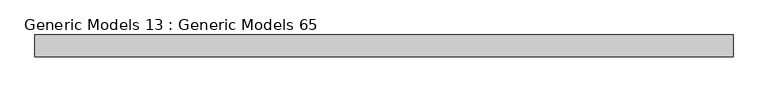
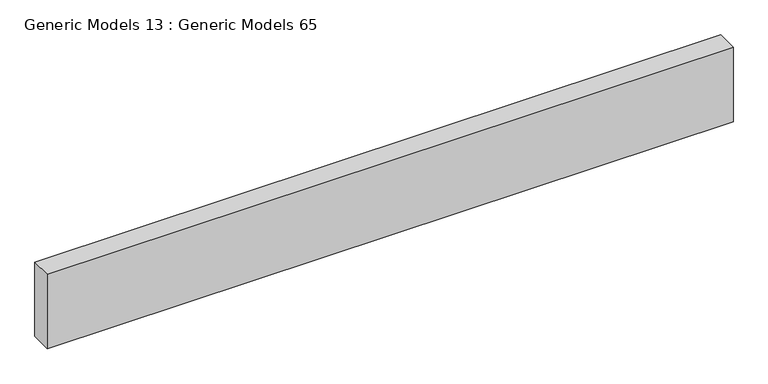
"""IFC4 building model written with IfcOpenShell, lengths in millimetres: proxy geometry, Generic Models 13 : Generic Models 65."""

from ifc_helpers import new_model, si_unit, frame, origin, place, context, project, spatial, polyline, outline, extrude, source, transform, mapped, element, save


def generic_models_13_generic_models_65_9e643fb9(model_context):
    return source(origin(), model_context, "Body", "SweptSolid", [
        extrude(outline(polyline([(49128.3625, 592.1375), (49128.3625, 630.2375), (50347.5625, 630.2375), (50347.5625, 592.1375), (49128.3625, 592.1375)])), frame((0.0, 0.0, 5507.83125), z_axis=(0.0, 0.0, 1.0), x_axis=(1.0, 0.0, 0.0)), (0.0, 0.0, 1.0), 139.7),
    ])


if __name__ == "__main__":
    model = new_model("IFC4")
    model_context = context("Model", 3, world=origin())
    ifc_project = project(units=[si_unit("LENGTHUNIT", "METRE", prefix="MILLI")], contexts=[model_context])
    site = spatial("IfcSite", under=ifc_project)
    building = spatial("IfcBuilding", under=site)
    placement = place(None, origin())
    generic_models_13_generic_models_65_shape = generic_models_13_generic_models_65_9e643fb9(model_context)
    element("IfcBuildingElementProxy", 1, Name="Generic Models 13 : Generic Models 65", ObjectType="Generic Models 13 : Generic Models 65", at=placement, inside=building, context=model_context, shape_type="MappedRepresentation", body=[
        mapped(generic_models_13_generic_models_65_shape, transform((0.0, 0.0, 0.0), x_axis=(1.0, 0.0, 0.0), y_axis=(0.0, 1.0, 0.0), z_axis=(0.0, 0.0, 1.0))),
    ])
    save(model, "model.ifc")

# Revit data of these elements
# Element 1 (IfcBuildingElementProxy, "Generic Models 13 : Generic Models 65")
#   Materials on its faces: "WOOD JOIST AS SPECIFIED"
# Materials
#   "WOOD JOIST AS SPECIFIED": class "Wood", colour RGB 234 198 147, transparency 0, Description = "Pinus Echinata", Cost = 0
